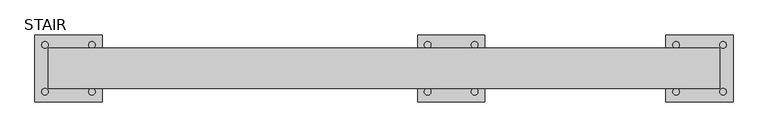
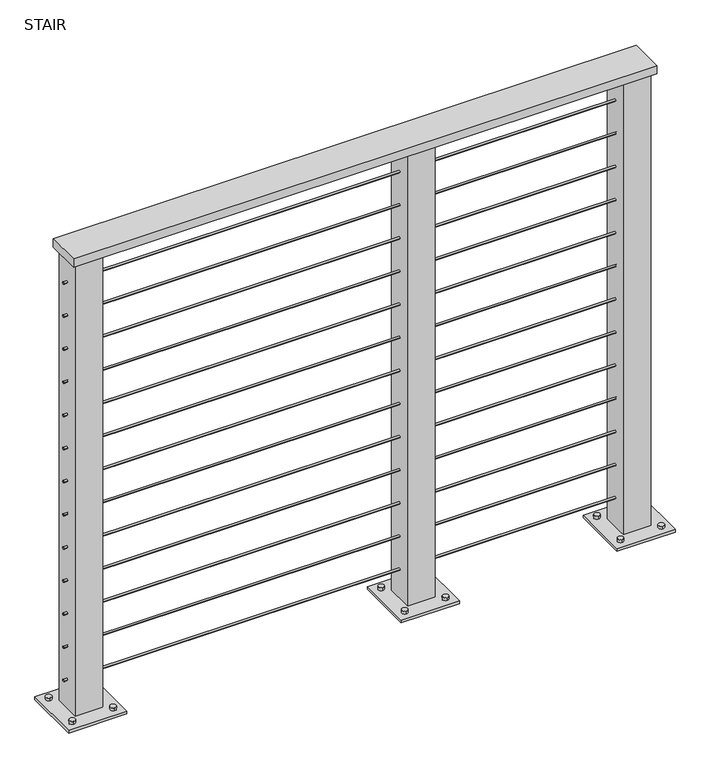
"""IFC4 building model written with IfcOpenShell, lengths in millimetres: railing geometry, STAIR."""

from ifc_helpers import new_model, si_unit, point, frame, frame_2d, origin, place, context, project, spatial, polyline, circle_curve, trimmed, segment, composite_curve, outline, extrude, source, transform, mapped, element, save


def stair_aa23c06f(model_context):
    return source(origin(), model_context, "Body", "SweptSolid", [
        extrude(outline(polyline([(27054.9620052, 5821.2594438), (27054.9620052, 5897.4594438), (28324.9620052, 5897.4594438), (28324.9620052, 5821.2594438), (27054.9620052, 5821.2594438)])), frame((0.0, 0.0, 3851.275), z_axis=(0.0, 0.0, 1.0), x_axis=(1.0, 0.0, 0.0)), (0.0, 0.0, 1.0), 19.05),
        extrude(outline(composite_curve([segment(trimmed(circle_curve(frame_2d((5859.3594438, 3791.74375)), 2.38125), [point((5861.7406938, 3791.74375))], [point((5856.9781938, 3791.74375))], False, "CARTESIAN"), True, "CONTINUOUS"), segment(trimmed(circle_curve(frame_2d((5859.3594438, 3791.74375)), 2.38125), [point((5856.9781938, 3791.74375))], [point((5861.7406938, 3791.74375))], False, "CARTESIAN"), True, "CONTINUOUS")], self_intersect=False)), frame((27054.9620052, 0.0, 0.0), z_axis=(1.0, 0.0, 0.0), x_axis=(0.0, 1.0, 0.0)), (0.0, 0.0, 1.0), 1270.0),
        extrude(outline(composite_curve([segment(trimmed(circle_curve(frame_2d((5859.3594438, 3715.54375)), 2.38125), [point((5861.7406938, 3715.54375))], [point((5856.9781938, 3715.54375))], False, "CARTESIAN"), True, "CONTINUOUS"), segment(trimmed(circle_curve(frame_2d((5859.3594438, 3715.54375)), 2.38125), [point((5856.9781938, 3715.54375))], [point((5861.7406938, 3715.54375))], False, "CARTESIAN"), True, "CONTINUOUS")], self_intersect=False)), frame((27054.9620052, 0.0, 0.0), z_axis=(1.0, 0.0, 0.0), x_axis=(0.0, 1.0, 0.0)), (0.0, 0.0, 1.0), 1270.0),
        extrude(outline(composite_curve([segment(trimmed(circle_curve(frame_2d((5859.3594438, 3639.34375)), 2.38125), [point((5861.7406938, 3639.34375))], [point((5856.9781938, 3639.34375))], False, "CARTESIAN"), True, "CONTINUOUS"), segment(trimmed(circle_curve(frame_2d((5859.3594438, 3639.34375)), 2.38125), [point((5856.9781938, 3639.34375))], [point((5861.7406938, 3639.34375))], False, "CARTESIAN"), True, "CONTINUOUS")], self_intersect=False)), frame((27054.9620052, 0.0, 0.0), z_axis=(1.0, 0.0, 0.0), x_axis=(0.0, 1.0, 0.0)), (0.0, 0.0, 1.0), 1270.0),
        extrude(outline(composite_curve([segment(trimmed(circle_curve(frame_2d((5859.3594438, 3563.14375)), 2.38125), [point((5861.7406938, 3563.14375))], [point((5856.9781938, 3563.14375))], False, "CARTESIAN"), True, "CONTINUOUS"), segment(trimmed(circle_curve(frame_2d((5859.3594438, 3563.14375)), 2.38125), [point((5856.9781938, 3563.14375))], [point((5861.7406938, 3563.14375))], False, "CARTESIAN"), True, "CONTINUOUS")], self_intersect=False)), frame((27054.9620052, 0.0, 0.0), z_axis=(1.0, 0.0, 0.0), x_axis=(0.0, 1.0, 0.0)), (0.0, 0.0, 1.0), 1270.0),
        extrude(outline(composite_curve([segment(trimmed(circle_curve(frame_2d((5859.3594438, 3486.94375)), 2.38125), [point((5861.7406938, 3486.94375))], [point((5856.9781938, 3486.94375))], False, "CARTESIAN"), True, "CONTINUOUS"), segment(trimmed(circle_curve(frame_2d((5859.3594438, 3486.94375)), 2.38125), [point((5856.9781938, 3486.94375))], [point((5861.7406938, 3486.94375))], False, "CARTESIAN"), True, "CONTINUOUS")], self_intersect=False)), frame((27054.9620052, 0.0, 0.0), z_axis=(1.0, 0.0, 0.0), x_axis=(0.0, 1.0, 0.0)), (0.0, 0.0, 1.0), 1270.0),
        extrude(outline(composite_curve([segment(trimmed(circle_curve(frame_2d((5859.3594438, 3410.74375)), 2.38125), [point((5861.7406938, 3410.74375))], [point((5856.9781938, 3410.74375))], False, "CARTESIAN"), True, "CONTINUOUS"), segment(trimmed(circle_curve(frame_2d((5859.3594438, 3410.74375)), 2.38125), [point((5856.9781938, 3410.74375))], [point((5861.7406938, 3410.74375))], False, "CARTESIAN"), True, "CONTINUOUS")], self_intersect=False)), frame((27054.9620052, 0.0, 0.0), z_axis=(1.0, 0.0, 0.0), x_axis=(0.0, 1.0, 0.0)), (0.0, 0.0, 1.0), 1270.0),
        extrude(outline(composite_curve([segment(trimmed(circle_curve(frame_2d((5859.3594438, 3334.54375)), 2.38125), [point((5861.7406938, 3334.54375))], [point((5856.9781938, 3334.54375))], False, "CARTESIAN"), True, "CONTINUOUS"), segment(trimmed(circle_curve(frame_2d((5859.3594438, 3334.54375)), 2.38125), [point((5856.9781938, 3334.54375))], [point((5861.7406938, 3334.54375))], False, "CARTESIAN"), True, "CONTINUOUS")], self_intersect=False)), frame((27054.9620052, 0.0, 0.0), z_axis=(1.0, 0.0, 0.0), x_axis=(0.0, 1.0, 0.0)), (0.0, 0.0, 1.0), 1270.0),
        extrude(outline(composite_curve([segment(trimmed(circle_curve(frame_2d((5859.3594438, 3258.34375)), 2.38125), [point((5861.7406938, 3258.34375))], [point((5856.9781938, 3258.34375))], False, "CARTESIAN"), True, "CONTINUOUS"), segment(trimmed(circle_curve(frame_2d((5859.3594438, 3258.34375)), 2.38125), [point((5856.9781938, 3258.34375))], [point((5861.7406938, 3258.34375))], False, "CARTESIAN"), True, "CONTINUOUS")], self_intersect=False)), frame((27054.9620052, 0.0, 0.0), z_axis=(1.0, 0.0, 0.0), x_axis=(0.0, 1.0, 0.0)), (0.0, 0.0, 1.0), 1270.0),
        extrude(outline(composite_curve([segment(trimmed(circle_curve(frame_2d((5859.3594438, 3182.14375)), 2.38125), [point((5861.7406938, 3182.14375))], [point((5856.9781938, 3182.14375))], False, "CARTESIAN"), True, "CONTINUOUS"), segment(trimmed(circle_curve(frame_2d((5859.3594438, 3182.14375)), 2.38125), [point((5856.9781938, 3182.14375))], [point((5861.7406938, 3182.14375))], False, "CARTESIAN"), True, "CONTINUOUS")], self_intersect=False)), frame((27054.9620052, 0.0, 0.0), z_axis=(1.0, 0.0, 0.0), x_axis=(0.0, 1.0, 0.0)), (0.0, 0.0, 1.0), 1270.0),
        extrude(outline(composite_curve([segment(trimmed(circle_curve(frame_2d((5859.3594438, 3105.94375)), 2.38125), [point((5861.7406938, 3105.94375))], [point((5856.9781938, 3105.94375))], False, "CARTESIAN"), True, "CONTINUOUS"), segment(trimmed(circle_curve(frame_2d((5859.3594438, 3105.94375)), 2.38125), [point((5856.9781938, 3105.94375))], [point((5861.7406938, 3105.94375))], False, "CARTESIAN"), True, "CONTINUOUS")], self_intersect=False)), frame((27054.9620052, 0.0, 0.0), z_axis=(1.0, 0.0, 0.0), x_axis=(0.0, 1.0, 0.0)), (0.0, 0.0, 1.0), 1270.0),
        extrude(outline(composite_curve([segment(trimmed(circle_curve(frame_2d((5859.3594438, 3029.74375)), 2.38125), [point((5861.7406938, 3029.74375))], [point((5856.9781938, 3029.74375))], False, "CARTESIAN"), True, "CONTINUOUS"), segment(trimmed(circle_curve(frame_2d((5859.3594438, 3029.74375)), 2.38125), [point((5856.9781938, 3029.74375))], [point((5861.7406938, 3029.74375))], False, "CARTESIAN"), True, "CONTINUOUS")], self_intersect=False)), frame((27054.9620052, 0.0, 0.0), z_axis=(1.0, 0.0, 0.0), x_axis=(0.0, 1.0, 0.0)), (0.0, 0.0, 1.0), 1270.0),
        extrude(outline(composite_curve([segment(trimmed(circle_curve(frame_2d((5859.3594438, 2953.54375)), 2.38125), [point((5861.7406938, 2953.54375))], [point((5856.9781938, 2953.54375))], False, "CARTESIAN"), True, "CONTINUOUS"), segment(trimmed(circle_curve(frame_2d((5859.3594438, 2953.54375)), 2.38125), [point((5856.9781938, 2953.54375))], [point((5861.7406938, 2953.54375))], False, "CARTESIAN"), True, "CONTINUOUS")], self_intersect=False)), frame((27054.9620052, 0.0, 0.0), z_axis=(1.0, 0.0, 0.0), x_axis=(0.0, 1.0, 0.0)), (0.0, 0.0, 1.0), 1270.0),
        extrude(outline(composite_curve([segment(trimmed(circle_curve(frame_2d((5859.3594438, 2877.34375)), 2.38125), [point((5861.7406938, 2877.34375))], [point((5856.9781938, 2877.34375))], False, "CARTESIAN"), True, "CONTINUOUS"), segment(trimmed(circle_curve(frame_2d((5859.3594438, 2877.34375)), 2.38125), [point((5856.9781938, 2877.34375))], [point((5861.7406938, 2877.34375))], False, "CARTESIAN"), True, "CONTINUOUS")], self_intersect=False)), frame((27054.9620052, 0.0, 0.0), z_axis=(1.0, 0.0, 0.0), x_axis=(0.0, 1.0, 0.0)), (0.0, 0.0, 1.0), 1270.0),
        extrude(outline(composite_curve([segment(trimmed(circle_curve(frame_2d((27772.5120052, 5814.9094438)), 6.35), [point((27772.5120052, 5808.5594438))], [point((27772.5120052, 5821.2594438))], False, "CARTESIAN"), True, "CONTINUOUS"), segment(trimmed(circle_curve(frame_2d((27772.5120052, 5814.9094438)), 6.35), [point((27772.5120052, 5821.2594438))], [point((27772.5120052, 5808.5594438))], False, "CARTESIAN"), True, "CONTINUOUS")], self_intersect=False)), frame((0.0, 0.0, 2803.525), z_axis=(0.0, 0.0, 1.0), x_axis=(1.0, 0.0, 0.0)), (0.0, 0.0, 1.0), 12.7),
        extrude(outline(composite_curve([segment(trimmed(circle_curve(frame_2d((27772.5120052, 5903.8094438)), 6.35), [point((27772.5120052, 5897.4594438))], [point((27772.5120052, 5910.1594438))], False, "CARTESIAN"), True, "CONTINUOUS"), segment(trimmed(circle_curve(frame_2d((27772.5120052, 5903.8094438)), 6.35), [point((27772.5120052, 5910.1594438))], [point((27772.5120052, 5897.4594438))], False, "CARTESIAN"), True, "CONTINUOUS")], self_intersect=False)), frame((0.0, 0.0, 2803.525), z_axis=(0.0, 0.0, 1.0), x_axis=(1.0, 0.0, 0.0)), (0.0, 0.0, 1.0), 12.7),
        extrude(outline(composite_curve([segment(trimmed(circle_curve(frame_2d((27861.4120052, 5814.9094438)), 6.35), [point((27861.4120052, 5808.5594438))], [point((27861.4120052, 5821.2594438))], False, "CARTESIAN"), True, "CONTINUOUS"), segment(trimmed(circle_curve(frame_2d((27861.4120052, 5814.9094438)), 6.35), [point((27861.4120052, 5821.2594438))], [point((27861.4120052, 5808.5594438))], False, "CARTESIAN"), True, "CONTINUOUS")], self_intersect=False)), frame((0.0, 0.0, 2803.525), z_axis=(0.0, 0.0, 1.0), x_axis=(1.0, 0.0, 0.0)), (0.0, 0.0, 1.0), 12.7),
        extrude(outline(composite_curve([segment(trimmed(circle_curve(frame_2d((27861.4120052, 5903.8094438)), 6.35), [point((27861.4120052, 5897.4594438))], [point((27861.4120052, 5910.1594438))], False, "CARTESIAN"), True, "CONTINUOUS"), segment(trimmed(circle_curve(frame_2d((27861.4120052, 5903.8094438)), 6.35), [point((27861.4120052, 5910.1594438))], [point((27861.4120052, 5897.4594438))], False, "CARTESIAN"), True, "CONTINUOUS")], self_intersect=False)), frame((0.0, 0.0, 2803.525), z_axis=(0.0, 0.0, 1.0), x_axis=(1.0, 0.0, 0.0)), (0.0, 0.0, 1.0), 12.7),
        extrude(outline(polyline([(27753.4620052, 5922.8594438), (27880.4620052, 5922.8594438), (27880.4620052, 5795.8594438), (27753.4620052, 5795.8594438), (27753.4620052, 5922.8594438)])), frame((0.0, 0.0, 2803.525), z_axis=(0.0, 0.0, 1.0), x_axis=(1.0, 0.0, 0.0)), (0.0, 0.0, 1.0), 6.35),
        extrude(outline(polyline([(27786.7995052, 5889.5219438), (27847.1245052, 5889.5219438), (27847.1245052, 5829.1969438), (27786.7995052, 5829.1969438), (27786.7995052, 5889.5219438)]), holes=[polyline([(27793.1495052, 5883.1719438), (27793.1495052, 5835.5469438), (27840.7745052, 5835.5469438), (27840.7745052, 5883.1719438), (27793.1495052, 5883.1719438)])]), frame((0.0, 0.0, 2803.525), z_axis=(0.0, 0.0, 1.0), x_axis=(1.0, 0.0, 0.0)), (0.0, 0.0, 1.0), 1047.75),
        extrude(outline(composite_curve([segment(trimmed(circle_curve(frame_2d((28242.4120052, 5814.9094438)), 6.35), [point((28242.4120052, 5808.5594438))], [point((28242.4120052, 5821.2594438))], False, "CARTESIAN"), True, "CONTINUOUS"), segment(trimmed(circle_curve(frame_2d((28242.4120052, 5814.9094438)), 6.35), [point((28242.4120052, 5821.2594438))], [point((28242.4120052, 5808.5594438))], False, "CARTESIAN"), True, "CONTINUOUS")], self_intersect=False)), frame((0.0, 0.0, 2803.525), z_axis=(0.0, 0.0, 1.0), x_axis=(1.0, 0.0, 0.0)), (0.0, 0.0, 1.0), 12.7),
        extrude(outline(composite_curve([segment(trimmed(circle_curve(frame_2d((28242.4120052, 5903.8094438)), 6.35), [point((28242.4120052, 5897.4594438))], [point((28242.4120052, 5910.1594438))], False, "CARTESIAN"), True, "CONTINUOUS"), segment(trimmed(circle_curve(frame_2d((28242.4120052, 5903.8094438)), 6.35), [point((28242.4120052, 5910.1594438))], [point((28242.4120052, 5897.4594438))], False, "CARTESIAN"), True, "CONTINUOUS")], self_intersect=False)), frame((0.0, 0.0, 2803.525), z_axis=(0.0, 0.0, 1.0), x_axis=(1.0, 0.0, 0.0)), (0.0, 0.0, 1.0), 12.7),
        extrude(outline(composite_curve([segment(trimmed(circle_curve(frame_2d((28331.3120052, 5814.9094438)), 6.35), [point((28331.3120052, 5808.5594438))], [point((28331.3120052, 5821.2594438))], False, "CARTESIAN"), True, "CONTINUOUS"), segment(trimmed(circle_curve(frame_2d((28331.3120052, 5814.9094438)), 6.35), [point((28331.3120052, 5821.2594438))], [point((28331.3120052, 5808.5594438))], False, "CARTESIAN"), True, "CONTINUOUS")], self_intersect=False)), frame((0.0, 0.0, 2803.525), z_axis=(0.0, 0.0, 1.0), x_axis=(1.0, 0.0, 0.0)), (0.0, 0.0, 1.0), 12.7),
        extrude(outline(composite_curve([segment(trimmed(circle_curve(frame_2d((28331.3120052, 5903.8094438)), 6.35), [point((28331.3120052, 5897.4594438))], [point((28331.3120052, 5910.1594438))], False, "CARTESIAN"), True, "CONTINUOUS"), segment(trimmed(circle_curve(frame_2d((28331.3120052, 5903.8094438)), 6.35), [point((28331.3120052, 5910.1594438))], [point((28331.3120052, 5897.4594438))], False, "CARTESIAN"), True, "CONTINUOUS")], self_intersect=False)), frame((0.0, 0.0, 2803.525), z_axis=(0.0, 0.0, 1.0), x_axis=(1.0, 0.0, 0.0)), (0.0, 0.0, 1.0), 12.7),
        extrude(outline(polyline([(28223.3620052, 5922.8594438), (28350.3620052, 5922.8594438), (28350.3620052, 5795.8594438), (28223.3620052, 5795.8594438), (28223.3620052, 5922.8594438)])), frame((0.0, 0.0, 2803.525), z_axis=(0.0, 0.0, 1.0), x_axis=(1.0, 0.0, 0.0)), (0.0, 0.0, 1.0), 6.35),
        extrude(outline(polyline([(28256.6995052, 5889.5219438), (28317.0245052, 5889.5219438), (28317.0245052, 5829.1969438), (28256.6995052, 5829.1969438), (28256.6995052, 5889.5219438)]), holes=[polyline([(28263.0495052, 5883.1719438), (28263.0495052, 5835.5469438), (28310.6745052, 5835.5469438), (28310.6745052, 5883.1719438), (28263.0495052, 5883.1719438)])]), frame((0.0, 0.0, 2803.525), z_axis=(0.0, 0.0, 1.0), x_axis=(1.0, 0.0, 0.0)), (0.0, 0.0, 1.0), 1047.75),
        extrude(outline(composite_curve([segment(trimmed(circle_curve(frame_2d((27048.6120052, 5814.9094438)), 6.35), [point((27048.6120052, 5808.5594438))], [point((27048.6120052, 5821.2594438))], False, "CARTESIAN"), True, "CONTINUOUS"), segment(trimmed(circle_curve(frame_2d((27048.6120052, 5814.9094438)), 6.35), [point((27048.6120052, 5821.2594438))], [point((27048.6120052, 5808.5594438))], False, "CARTESIAN"), True, "CONTINUOUS")], self_intersect=False)), frame((0.0, 0.0, 2803.525), z_axis=(0.0, 0.0, 1.0), x_axis=(1.0, 0.0, 0.0)), (0.0, 0.0, 1.0), 12.7),
        extrude(outline(composite_curve([segment(trimmed(circle_curve(frame_2d((27048.6120052, 5903.8094438)), 6.35), [point((27048.6120052, 5897.4594438))], [point((27048.6120052, 5910.1594438))], False, "CARTESIAN"), True, "CONTINUOUS"), segment(trimmed(circle_curve(frame_2d((27048.6120052, 5903.8094438)), 6.35), [point((27048.6120052, 5910.1594438))], [point((27048.6120052, 5897.4594438))], False, "CARTESIAN"), True, "CONTINUOUS")], self_intersect=False)), frame((0.0, 0.0, 2803.525), z_axis=(0.0, 0.0, 1.0), x_axis=(1.0, 0.0, 0.0)), (0.0, 0.0, 1.0), 12.7),
        extrude(outline(composite_curve([segment(trimmed(circle_curve(frame_2d((27137.5120052, 5814.9094438)), 6.35), [point((27137.5120052, 5808.5594438))], [point((27137.5120052, 5821.2594438))], False, "CARTESIAN"), True, "CONTINUOUS"), segment(trimmed(circle_curve(frame_2d((27137.5120052, 5814.9094438)), 6.35), [point((27137.5120052, 5821.2594438))], [point((27137.5120052, 5808.5594438))], False, "CARTESIAN"), True, "CONTINUOUS")], self_intersect=False)), frame((0.0, 0.0, 2803.525), z_axis=(0.0, 0.0, 1.0), x_axis=(1.0, 0.0, 0.0)), (0.0, 0.0, 1.0), 12.7),
        extrude(outline(composite_curve([segment(trimmed(circle_curve(frame_2d((27137.5120052, 5903.8094438)), 6.35), [point((27137.5120052, 5897.4594438))], [point((27137.5120052, 5910.1594438))], False, "CARTESIAN"), True, "CONTINUOUS"), segment(trimmed(circle_curve(frame_2d((27137.5120052, 5903.8094438)), 6.35), [point((27137.5120052, 5910.1594438))], [point((27137.5120052, 5897.4594438))], False, "CARTESIAN"), True, "CONTINUOUS")], self_intersect=False)), frame((0.0, 0.0, 2803.525), z_axis=(0.0, 0.0, 1.0), x_axis=(1.0, 0.0, 0.0)), (0.0, 0.0, 1.0), 12.7),
        extrude(outline(polyline([(27029.5620052, 5922.8594438), (27156.5620052, 5922.8594438), (27156.5620052, 5795.8594438), (27029.5620052, 5795.8594438), (27029.5620052, 5922.8594438)])), frame((0.0, 0.0, 2803.525), z_axis=(0.0, 0.0, 1.0), x_axis=(1.0, 0.0, 0.0)), (0.0, 0.0, 1.0), 6.35),
        extrude(outline(polyline([(27062.8995052, 5889.5219438), (27123.2245052, 5889.5219438), (27123.2245052, 5829.1969438), (27062.8995052, 5829.1969438), (27062.8995052, 5889.5219438)]), holes=[polyline([(27069.2495052, 5883.1719438), (27069.2495052, 5835.5469438), (27116.8745052, 5835.5469438), (27116.8745052, 5883.1719438), (27069.2495052, 5883.1719438)])]), frame((0.0, 0.0, 2803.525), z_axis=(0.0, 0.0, 1.0), x_axis=(1.0, 0.0, 0.0)), (0.0, 0.0, 1.0), 1047.75),
    ])


if __name__ == "__main__":
    model = new_model("IFC4")
    model_context = context("Model", 3, world=origin())
    ifc_project = project(units=[si_unit("LENGTHUNIT", "METRE", prefix="MILLI")], contexts=[model_context])
    site = spatial("IfcSite", under=ifc_project)
    building = spatial("IfcBuilding", under=site)
    placement = place(None, origin())
    stair_shape = stair_aa23c06f(model_context)
    element("IfcRailing", 1, ObjectType="STAIR", at=placement, inside=building, context=model_context, shape_type="MappedRepresentation", body=[
        mapped(stair_shape, transform((0.0, 0.0, 0.0), x_axis=(1.0, 0.0, 0.0), y_axis=(0.0, 1.0, 0.0), z_axis=(0.0, 0.0, 1.0))),
    ])
    save(model, "model.ifc")

# Revit data of these elements
# Element 1 (IfcRailing, "STAIR")
#   Materials on its faces: "2 1/2\" X 2 1/2\" ALUM. SQUARE POST (38\" O.C. MAX)", "WIRE RAILING (3\" O.C.)", "ALUM. PLATE TOP RAIL"
# Materials
#   "2 1/2\" X 2 1/2\" ALUM. SQUARE POST (38\" O.C. MAX)": class "Metal", colour RGB 244 244 244, transparency 0, Manufacturer = "Kawneer", URL = "http://www.kawneer.com/kawneer/north_america/en/home.asp", Cost = 0
#   "WIRE RAILING (3\" O.C.)": class "Metal", colour RGB 244 244 244, transparency 0, Manufacturer = "Kawneer", URL = "http://www.kawneer.com/kawneer/north_america/en/home.asp", Cost = 0
#   "ALUM. PLATE TOP RAIL": class "Metal", colour RGB 244 244 244, transparency 0, Manufacturer = "Kawneer", URL = "http://www.kawneer.com/kawneer/north_america/en/home.asp", Cost = 0
